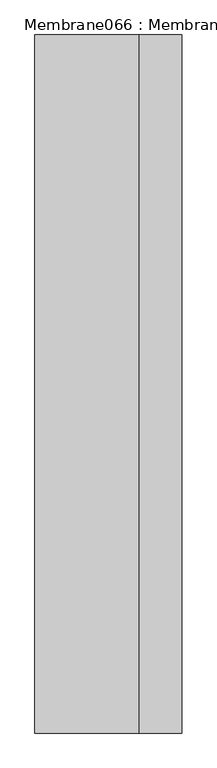
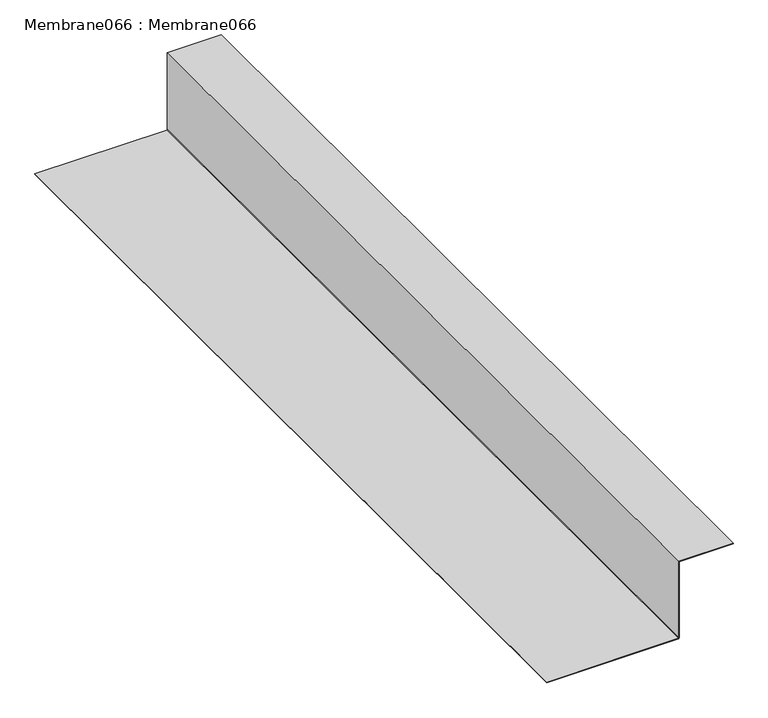
"""IFC4 building model written with IfcOpenShell, lengths in millimetres: proxy geometry, Membrane066 : Membrane066."""

from ifc_helpers import new_model, si_unit, frame, origin, place, context, project, spatial, polyline, outline, extrude, source, transform, mapped, element, save


def membrane066_membrane066_3455b8cb(model_context):
    return source(origin(), model_context, "Body", "SweptSolid", [
        extrude(outline(polyline([(42574.9034828, 5754.1278536), (42573.7128578, 5754.1278536), (42573.7128578, 6052.0153885), (42575.5508814, 6053.853412), (42757.5078125, 6053.853412), (42757.5078125, 6174.7895508), (42758.6984375, 6174.7895508), (42758.6984375, 6052.662787), (42576.0440544, 6052.662787), (42574.9034828, 6051.5222154), (42574.9034828, 5754.1278536)])), frame((0.0, -1052.8906574, 0.0), z_axis=(0.0, 1.0, 0.0), x_axis=(0.0, 0.0, 1.0)), (0.0, 0.0, 1.0), 1999.85),
    ])


if __name__ == "__main__":
    model = new_model("IFC4")
    model_context = context("Model", 3, world=origin())
    ifc_project = project(units=[si_unit("LENGTHUNIT", "METRE", prefix="MILLI")], contexts=[model_context])
    site = spatial("IfcSite", under=ifc_project)
    building = spatial("IfcBuilding", under=site)
    placement = place(None, origin())
    membrane066_membrane066_shape = membrane066_membrane066_3455b8cb(model_context)
    element("IfcBuildingElementProxy", 1, Name="Membrane066 : Membrane066", ObjectType="Membrane066 : Membrane066", at=placement, inside=building, context=model_context, shape_type="MappedRepresentation", body=[
        mapped(membrane066_membrane066_shape, transform((0.0, 0.0, 0.0), x_axis=(1.0, 0.0, 0.0), y_axis=(0.0, 1.0, 0.0), z_axis=(0.0, 0.0, 1.0))),
    ])
    save(model, "model.ifc")

# Revit data of these elements
# Type "Membrane066 : Membrane066"
#   NameOverride = "Membrane066"
# Element 1 (IfcBuildingElementProxy, "Membrane066 : Membrane066")
#   Materials on its faces: "ASPHALT SATURATED ORGANIC FELT @ ROOF"
# Materials
#   "ASPHALT SATURATED ORGANIC FELT @ ROOF": class "Unassigned", colour RGB 85 170 127, transparency 0
